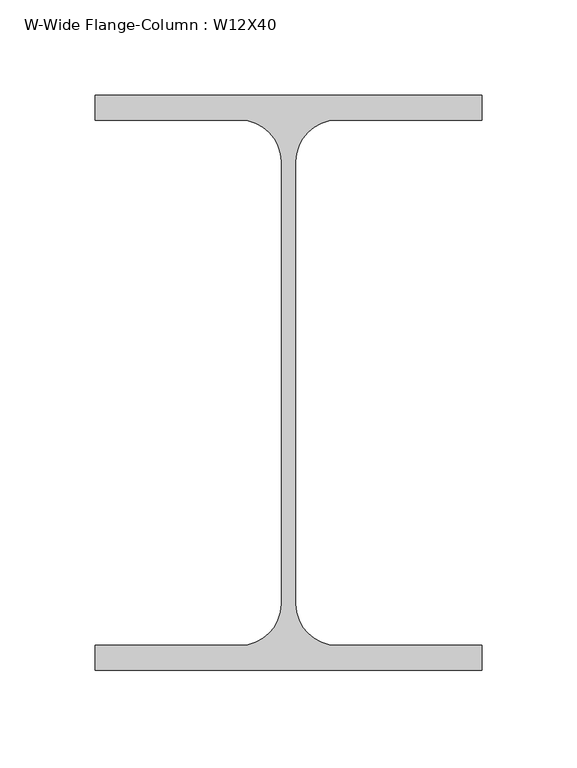
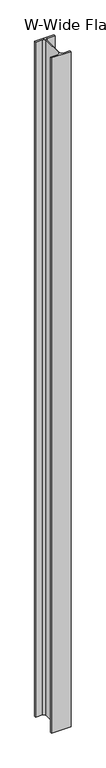
"""IFC4 building model written with IfcOpenShell, lengths in millimetres: column geometry, W-Wide Flange-Column : W12X40."""

from ifc_helpers import new_model, si_unit, point, frame, frame_2d, origin, place, context, project, spatial, polyline, circle_curve, trimmed, segment, composite_curve, outline, extrude, source, transform, mapped, element, save


def w_wide_flange_column_w12x40_e879ecb8(model_context):
    return source(origin(), model_context, "Body", "SweptSolid", [
        extrude(outline(composite_curve([segment(polyline([(101.727, 151.13), (101.727, 138.049), (25.5905, 138.049)]), True, "CONTINUOUS"), segment(trimmed(circle_curve(frame_2d((25.5905, 116.205)), 21.844), [point((25.5905, 138.049))], [point((3.7465, 116.205))], True, "CARTESIAN"), True, "CONTINUOUS"), segment(polyline([(3.7465, 116.205), (3.7465, -116.205)]), True, "CONTINUOUS"), segment(trimmed(circle_curve(frame_2d((25.5905, -116.205)), 21.844), [point((3.7465, -116.205))], [point((25.5905, -138.049))], True, "CARTESIAN"), True, "CONTINUOUS"), segment(polyline([(25.5905, -138.049), (101.727, -138.049), (101.727, -151.13), (-101.727, -151.13), (-101.727, -138.049), (-25.5905, -138.049)]), True, "CONTINUOUS"), segment(trimmed(circle_curve(frame_2d((-25.5905, -116.205)), 21.844), [point((-25.5905, -138.049))], [point((-3.7465, -116.205))], True, "CARTESIAN"), True, "CONTINUOUS"), segment(polyline([(-3.7465, -116.205), (-3.7465, 116.205)]), True, "CONTINUOUS"), segment(trimmed(circle_curve(frame_2d((-25.5905, 116.205)), 21.844), [point((-3.7465, 116.205))], [point((-25.5905, 138.049))], True, "CARTESIAN"), True, "CONTINUOUS"), segment(polyline([(-25.5905, 138.049), (-101.727, 138.049), (-101.727, 151.13), (101.727, 151.13)]), True, "CONTINUOUS")], self_intersect=False)), frame((0.0, 0.0, 8756.65), z_axis=(0.0, 0.0, 1.0), x_axis=(1.0, 0.0, 0.0)), (0.0, 0.0, 1.0), 7448.55),
    ])


if __name__ == "__main__":
    model = new_model("IFC4")
    model_context = context("Model", 3, world=origin())
    ifc_project = project(units=[si_unit("LENGTHUNIT", "METRE", prefix="MILLI")], contexts=[model_context])
    site = spatial("IfcSite", under=ifc_project)
    building = spatial("IfcBuilding", under=site)
    placement = place(None, origin())
    w_wide_flange_column_w12x40_shape = w_wide_flange_column_w12x40_e879ecb8(model_context)
    element("IfcColumn", 1, ObjectType="W-Wide Flange-Column : W12X40", at=placement, inside=building, context=model_context, shape_type="MappedRepresentation", body=[
        mapped(w_wide_flange_column_w12x40_shape, transform((0.0, 0.0, 0.0), x_axis=(1.0, 0.0, 0.0), y_axis=(0.0, 1.0, 0.0), z_axis=(0.0, 0.0, 1.0))),
    ])
    save(model, "model.ifc")

# Revit data of these elements
# Type "W-Wide Flange-Column : W12X40"
#   Assembly Code = "B10"
#   W = 40
#   bf = 0' - 8.01"
#   d = 0' - 11.9"
#   k = 0' - 1 3/8"
#   kr = 0' - 0.86"
#   tf = 0' - 0.515"
#   tw = 0' - 0.295"
#   A = 0.08125 SF
#   Structural Material [instance default] = Steel ASTM A992
# Element 1 (IfcColumn, "W-Wide Flange-Column : W12X40")
#   Materials on its faces: "Steel ASTM A992"
# Materials
#   "Steel ASTM A992": class "Metal", colour RGB 199 199 199, transparency 0, Description = "Structural steel 50ksi", Cost = 0
